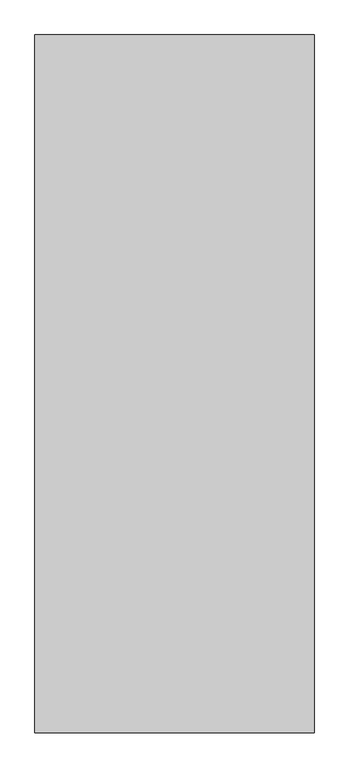
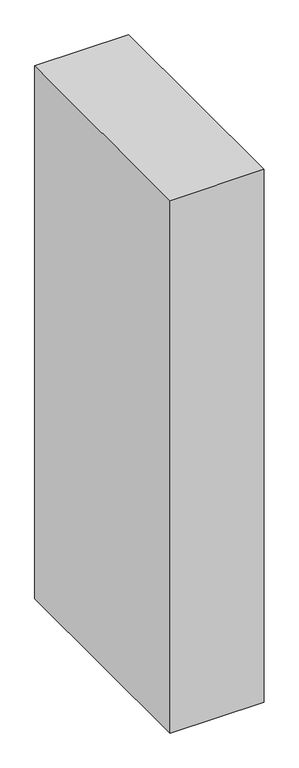
"""IFC4 building model written with IfcOpenShell, lengths in millimetres: proxy geometry, Space Planning Box_hec : Space Planning Box_hec."""

import ifcopenshell
import ifcopenshell.guid

model = None  # the IFC model being written
_history = None  # IfcOwnerHistory: only IFC2X3 demands one
_inside = {}  # id of a spatial element -> (the spatial element, [elements in it])
_under = {}  # id of a project, library or spatial element -> (it, [spatial elements below it])
_declared = {}  # id of a project -> (the project, [libraries it declares])
_typed = {}  # id of a type object -> (the type object, [elements of that type])
_made_of = {}  # id of a material, layer set ... -> (it, [elements and type objects made of it])


def new_model(schema):
    """Start an empty IFC model of exactly this schema.

    Asked for "IFC4X3", IfcOpenShell would pick the latest addendum, in which some entities
    have other attributes; the version numbers below select the first issue.
    IFC2X3 requires an IfcOwnerHistory on every rooted entity: one is made here for all.
    """
    global model, _history
    if schema == "IFC4X3":
        model = ifcopenshell.file(schema_version=(4, 3, 0, 0))
    else:
        model = ifcopenshell.file(schema=schema)
    _inside.clear()
    _under.clear()
    _declared.clear()
    _typed.clear()
    _made_of.clear()
    _history = None
    if model.schema == "IFC2X3":
        org = make("IfcOrganization", Name="unknown")
        user = make(
            "IfcPersonAndOrganization",
            ThePerson=make("IfcPerson", FamilyName="unknown"),
            TheOrganization=org,
        )
        app = make(
            "IfcApplication",
            ApplicationDeveloper=org,
            Version="unknown",
            ApplicationFullName="unknown",
            ApplicationIdentifier="unknown",
        )
        _history = make(
            "IfcOwnerHistory",
            OwningUser=user,
            OwningApplication=app,
            ChangeAction="ADDED",
            CreationDate=0,
        )
    return model


def make(cls, **values):
    """One entity of the class cls with the attributes given. An attribute that is None is left unset."""
    return model.create_entity(
        cls, **{name: value for name, value in values.items() if value is not None}
    )


def rooted(cls, **values):
    """An entity with a GlobalId (a new one), such as an element, a storey or a relation."""
    return make(cls, GlobalId=ifcopenshell.guid.new(), OwnerHistory=_history, **values)


def si_unit(unit_type, name, prefix=None):
    """IfcSIUnit, for example si_unit("LENGTHUNIT", "METRE", prefix="MILLI")."""
    return make("IfcSIUnit", UnitType=unit_type, Prefix=prefix, Name=name)


def assignment(units):
    """IfcUnitAssignment: the units of a project."""
    return None if units is None else make("IfcUnitAssignment", Units=units)


def point(xyz):
    """IfcCartesianPoint."""
    return None if xyz is None else make("IfcCartesianPoint", Coordinates=xyz)


def direction(xyz):
    """IfcDirection."""
    return None if xyz is None else make("IfcDirection", DirectionRatios=xyz)


def frame(location, z_axis=None, x_axis=None):
    """IfcAxis2Placement3D, a coordinate frame: its origin and axes. An axis left out is left unset."""
    return make(
        "IfcAxis2Placement3D",
        Location=point(location),
        Axis=direction(z_axis),
        RefDirection=direction(x_axis),
    )


def origin():
    """The frame at (0, 0, 0) with its axes left unset."""
    return frame((0.0, 0.0, 0.0))


def origin_with_axes():
    """The frame at (0, 0, 0) with the z axis (0, 0, 1) and the x axis (1, 0, 0) written out."""
    return frame((0.0, 0.0, 0.0), z_axis=(0.0, 0.0, 1.0), x_axis=(1.0, 0.0, 0.0))


def place(relative_to, where):
    """IfcLocalPlacement: puts the frame where relative to a parent placement (None: the world)."""
    return make(
        "IfcLocalPlacement", PlacementRelTo=relative_to, RelativePlacement=where
    )


def context(
    kind, dimensions, precision=None, world=None, true_north=None, identifier=None
):
    """IfcGeometricRepresentationContext, for example the 3D "Model" context."""
    return make(
        "IfcGeometricRepresentationContext",
        ContextIdentifier=identifier,
        ContextType=kind,
        CoordinateSpaceDimension=dimensions,
        Precision=precision,
        WorldCoordinateSystem=world,
        TrueNorth=true_north,
    )


def project(units=None, contexts=None):
    """IfcProject with its units and contexts."""
    return rooted(
        "IfcProject",
        Name="project",
        RepresentationContexts=contexts,
        UnitsInContext=assignment(units),
    )


def spatial(cls, under=None, at=None, **own):
    """A site, building, storey or space (cls), placed at a placement, below another one or the project."""
    s = rooted(cls, ObjectPlacement=at, **own)
    if under is not None:
        _under.setdefault(under.id(), (under, []))[1].append(s)
    return s


def polyline(points):
    """IfcPolyline through the points."""
    return make("IfcPolyline", Points=[point(p) for p in points])


def outline(outer, holes=None, kind="AREA"):
    """IfcArbitraryClosedProfileDef: a profile drawn as a closed curve; with holes, ...WithVoids."""
    if holes is None:
        return make("IfcArbitraryClosedProfileDef", ProfileType=kind, OuterCurve=outer)
    return make(
        "IfcArbitraryProfileDefWithVoids",
        ProfileType=kind,
        OuterCurve=outer,
        InnerCurves=holes,
    )


def extrude(swept, where, along, depth):
    """IfcExtrudedAreaSolid: the profile swept, set in the frame where, extruded along a direction by depth."""
    return make(
        "IfcExtrudedAreaSolid",
        SweptArea=swept,
        Position=where,
        ExtrudedDirection=direction(along),
        Depth=depth,
    )


def shape(context_of_items, identifier, shape_type, items):
    """IfcShapeRepresentation: the items that make up one representation, for example the "Body"."""
    return make(
        "IfcShapeRepresentation",
        ContextOfItems=context_of_items,
        RepresentationIdentifier=identifier,
        RepresentationType=shape_type,
        Items=items,
    )


def source(mapping_origin, context_of_items, identifier, shape_type, items):
    """IfcRepresentationMap: a shape defined once, which mapped items show again and again."""
    return make(
        "IfcRepresentationMap",
        MappingOrigin=mapping_origin,
        MappedRepresentation=shape(context_of_items, identifier, shape_type, items),
    )


def transform(
    local_origin,
    x_axis=None,
    y_axis=None,
    z_axis=None,
    scale=None,
    scale2=None,
    scale3=None,
    uniform=True,
):
    """IfcCartesianTransformationOperator3D, or its non-uniform kind. x_axis, y_axis, z_axis: its Axis1, 2, 3."""
    if uniform:
        return make(
            "IfcCartesianTransformationOperator3D",
            Axis1=direction(x_axis),
            Axis2=direction(y_axis),
            LocalOrigin=point(local_origin),
            Scale=scale,
            Axis3=direction(z_axis),
        )
    return make(
        "IfcCartesianTransformationOperator3DnonUniform",
        Axis1=direction(x_axis),
        Axis2=direction(y_axis),
        LocalOrigin=point(local_origin),
        Scale=scale,
        Axis3=direction(z_axis),
        Scale2=scale2,
        Scale3=scale3,
    )


def mapped(mapping_source, mapping_target):
    """IfcMappedItem: shows the shape of a source again, moved by a transform."""
    return make(
        "IfcMappedItem", MappingSource=mapping_source, MappingTarget=mapping_target
    )


def made_of(thing, what):
    """Note that an element or type object is made of a material, layer set ...; save() writes the relation."""
    if what is not None:
        _made_of.setdefault(what.id(), (what, []))[1].append(thing)
    return thing


def element(
    cls,
    number,
    at=None,
    inside=None,
    cuts=None,
    type_object=None,
    material=None,
    context=None,
    identifier="Body",
    shape_type=None,
    held_by="IfcProductDefinitionShape",
    body=None,
    shapes=None,
    **own,
):
    """One element of the class cls, such as IfcWall. Its Tag is "e" and its number.

    at: its placement. inside: the storey or other place that contains it. cuts: it is an
    opening in that element (IfcRelVoidsElement). A single representation is given by context,
    identifier, shape_type and body (its items); several are given by shapes. held_by: the class
    of the entity that holds the representations. save() writes the other relations.
    """
    e = rooted(cls, Tag="e%d" % number, ObjectPlacement=at, **own)
    if body is not None:
        shapes = [shape(context, identifier, shape_type, body)]
    if shapes is not None:
        e.Representation = make(held_by, Representations=shapes)
    if inside is not None:
        _inside.setdefault(inside.id(), (inside, []))[1].append(e)
    if cuts is not None:
        rooted(
            "IfcRelVoidsElement", RelatingBuildingElement=cuts, RelatedOpeningElement=e
        )
    if type_object is not None:
        _typed.setdefault(type_object.id(), (type_object, []))[1].append(e)
    return made_of(e, material)


def aggregate(whole, parts):
    """IfcRelAggregates: a whole, such as a stair, and the parts it consists of."""
    return rooted("IfcRelAggregates", RelatingObject=whole, RelatedObjects=parts)


def save(model, path):
    """Write the relations noted so far, then the file.

    IfcRelAggregates (storeys below a building ...), IfcRelContainedInSpatialStructure (elements
    in a storey), IfcRelDefinesByType, IfcRelAssociatesMaterial and IfcRelDeclares: one each for
    every whole, place, type object, material and project.
    """
    for whole, parts in _under.values():
        aggregate(whole, parts)
    for where, things in _inside.values():
        rooted(
            "IfcRelContainedInSpatialStructure",
            RelatedElements=things,
            RelatingStructure=where,
        )
    for kind, things in _typed.values():
        rooted("IfcRelDefinesByType", RelatedObjects=things, RelatingType=kind)
    for what, things in _made_of.values():
        rooted("IfcRelAssociatesMaterial", RelatedObjects=things, RelatingMaterial=what)
    for by, libraries in _declared.values():
        rooted("IfcRelDeclares", RelatingContext=by, RelatedDefinitions=libraries)
    model.write(path)


def generic_models_71e2440f(model_context):
    return source(origin(), model_context, "Body", "SweptSolid", [
        extrude(outline(polyline([(500.0, 1250.0), (500.0, -1250.0), (-500.0, -1250.0), (-500.0, 1250.0), (500.0, 1250.0)])), origin_with_axes(), (0.0, 0.0, 1.0), 6000.0),
    ])


if __name__ == "__main__":
    model = new_model("IFC4")
    model_context = context("Model", 3, world=origin())
    ifc_project = project(units=[si_unit("LENGTHUNIT", "METRE", prefix="MILLI")], contexts=[model_context])
    site = spatial("IfcSite", under=ifc_project)
    building = spatial("IfcBuilding", under=site)
    placement = place(None, origin())
    generic_models_shape = generic_models_71e2440f(model_context)
    element("IfcBuildingElementProxy", 1, Name="Space Planning Box_hec : Space Planning Box_hec", ObjectType="Space Planning Box_hec : Space Planning Box_hec", at=placement, inside=building, context=model_context, shape_type="MappedRepresentation", body=[
        mapped(generic_models_shape, transform((0.0, 0.0, 0.0), x_axis=(1.0, 0.0, 0.0), y_axis=(0.0, 1.0, 0.0), z_axis=(0.0, 0.0, 1.0))),
    ])
    save(model, "model.ifc")

# Revit data of these elements
# Type "Space Planning Box_hec : Space Planning Box_hec"
#   Type Comments = "..."
#   Room Name [instance default] = "?"
#   Interior Finish [instance default] = ""
#   Exterior Finish [instance default] = ""
#   Department [instance default] = ""
#   Assembly Code = "..."
#   Width [instance default] = 1524 mm
#   Program Area [instance default] = 0 m²
#   Length [instance default] = 1524 mm
#   Height [instance default] = 1524 mm
#   Area [instance default] = 2.32258 m²
#   Fill Color [instance default] = Cyan
#   Default Elevation = 0
# Element 1 (IfcBuildingElementProxy, "Space Planning Box_hec : Space Planning Box_hec")
#   Room Name = "Pipe Shaft"
#   Interior Finish = "NA"
#   Exterior Finish = "EF1"
#   Department = "HV"
#   Width = 1000 mm
#   Program Area = 2.5 m²
#   Length = 2500 mm
#   Height = 6000 mm
#   Area = 2.5 m²
#   Fill Color = Pink
#   Materials on its faces: "Pink"
# Materials
#   "Cyan": class "Generic", colour RGB 0 255 255, transparency 0.2, Cost = 0
#   "Pink": class "Generic", colour RGB 255 105 180, transparency 0.2, Cost = 0
